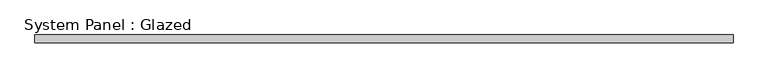
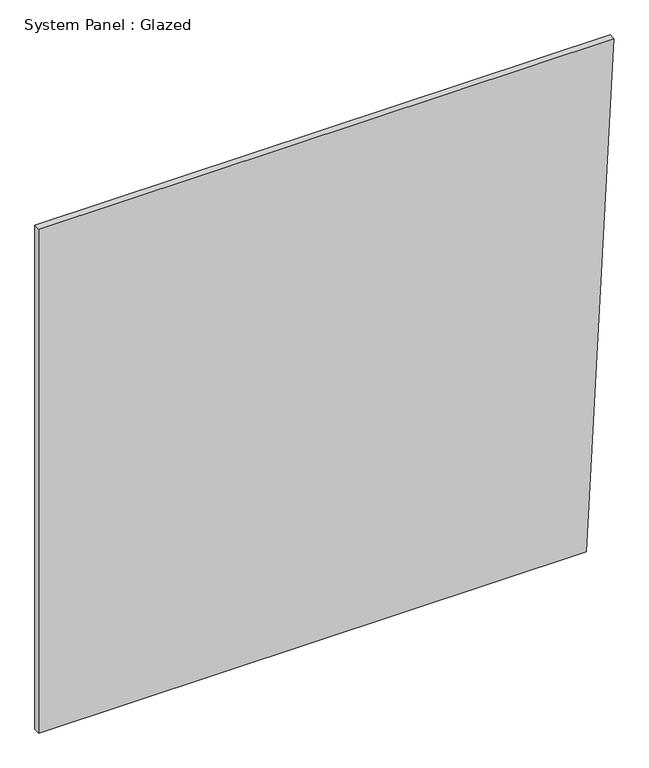
"""IFC4 building model written with IfcOpenShell, lengths in millimetres: plate geometry, System Panel : Glazed."""

from ifc_helpers import new_model, si_unit, frame, origin, place, context, project, spatial, polyline, outline, extrude, source, transform, mapped, element, save


def system_panel_glazed_3f2e0697(model_context):
    return source(origin(), model_context, "Body", "SweptSolid", [
        extrude(outline(polyline([(0.0, -1126.1853377), (0.0, 1017.0034845), (2086.1728929, 1126.1853377), (2086.1728929, -1126.1853377), (0.0, -1126.1853377)])), frame((0.0, -44.45, 0.0), z_axis=(0.0, 1.0, 0.0), x_axis=(0.0, 0.0, 1.0)), (0.0, 0.0, 1.0), 25.4),
    ])


if __name__ == "__main__":
    model = new_model("IFC4")
    model_context = context("Model", 3, world=origin())
    ifc_project = project(units=[si_unit("LENGTHUNIT", "METRE", prefix="MILLI")], contexts=[model_context])
    site = spatial("IfcSite", under=ifc_project)
    building = spatial("IfcBuilding", under=site)
    placement = place(None, origin())
    system_panel_glazed_shape = system_panel_glazed_3f2e0697(model_context)
    element("IfcPlate", 1, ObjectType="System Panel : Glazed", at=placement, inside=building, context=model_context, shape_type="MappedRepresentation", body=[
        mapped(system_panel_glazed_shape, transform((0.0, 0.0, 0.0), x_axis=(1.0, 0.0, 0.0), y_axis=(0.0, 1.0, 0.0), z_axis=(0.0, 0.0, 1.0))),
    ])
    save(model, "model.ifc")

# Revit data of these elements
# Type "System Panel : Glazed"
#   Construction Type Id = "GSP4R"
#   Analytic Construction = "1/8 in Pilkington single glazing"
#   Visual Light Transmittance = 0.9
#   Solar Heat Gain Coefficient = 0.86
#   Heat Transfer Coefficient (U) = 1.18115 BTU/(h·ft²·°F)
#   Define Thermal Properties by = 1
# Element 1 (IfcPlate, "System Panel : Glazed")
#   Materials on its faces: "Glass"
# Materials
#   "Glass": class "Glass", colour RGB 0 128 192, transparency 0.75, Description = "Soda Lime Glass", Cost = 0
